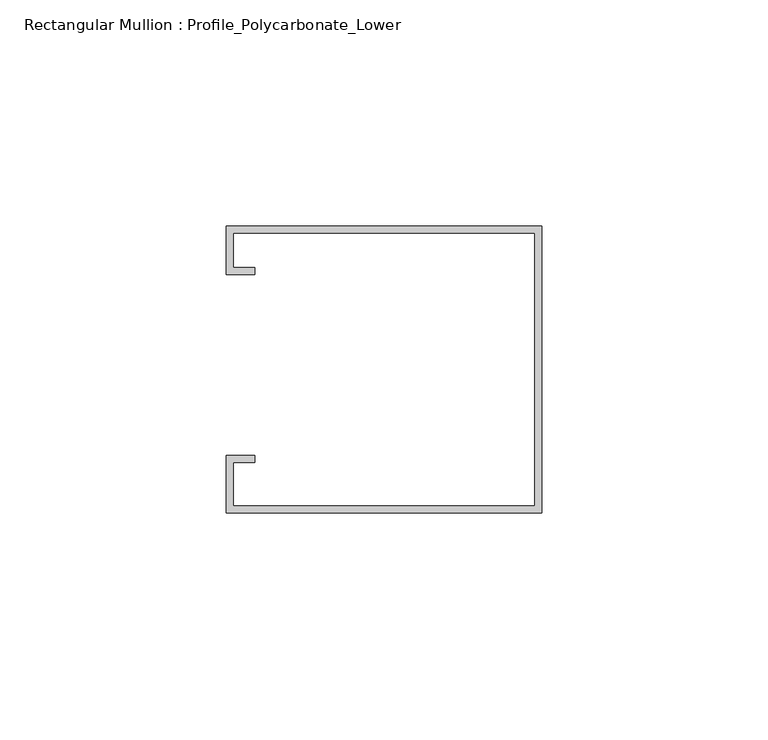
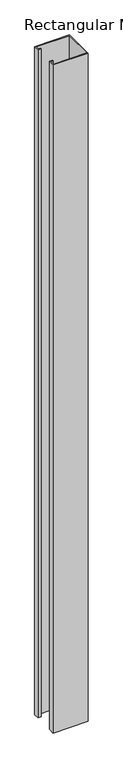
"""IFC4 building model written with IfcOpenShell, lengths in millimetres: member geometry, Rectangular Mullion : Profile_Polycarbonate_Lower."""

from ifc_helpers import new_model, si_unit, frame, origin, place, context, project, spatial, polyline, outline, extrude, source, transform, mapped, element, save


def rectangular_mullion_profile_polycarbonate_lower_301292b8(model_context):
    return source(origin(), model_context, "Body", "SweptSolid", [
        extrude(outline(polyline([(0.0, -32.7), (-69.85, -32.7), (-69.85, -20.0), (-63.5, -20.0), (-63.5, -21.5875), (-68.2625, -21.5875), (-68.2625, -31.1125), (-1.5875, -31.1125), (-1.5875, 29.2125), (-68.2625, 29.2125), (-68.2625, 21.5875), (-63.5, 21.5875), (-63.5, 20.0), (-69.85, 20.0), (-69.85, 30.8), (0.0, 30.8), (0.0, -32.7)])), frame((0.0, 0.0, -1409.7), z_axis=(0.0, 0.0, 1.0), x_axis=(1.0, 0.0, 0.0)), (0.0, 0.0, 1.0), 1409.7),
    ])


if __name__ == "__main__":
    model = new_model("IFC4")
    model_context = context("Model", 3, world=origin())
    ifc_project = project(units=[si_unit("LENGTHUNIT", "METRE", prefix="MILLI")], contexts=[model_context])
    site = spatial("IfcSite", under=ifc_project)
    building = spatial("IfcBuilding", under=site)
    placement = place(None, origin())
    rectangular_mullion_profile_polycarbonate_lower_shape = rectangular_mullion_profile_polycarbonate_lower_301292b8(model_context)
    element("IfcMember", 1, ObjectType="Rectangular Mullion : Profile_Polycarbonate_Lower", at=placement, inside=building, context=model_context, shape_type="MappedRepresentation", body=[
        mapped(rectangular_mullion_profile_polycarbonate_lower_shape, transform((0.0, 0.0, 0.0), x_axis=(1.0, 0.0, 0.0), y_axis=(0.0, 1.0, 0.0), z_axis=(0.0, 0.0, 1.0))),
    ])
    save(model, "model.ifc")

# Revit data of these elements
# Type "Rectangular Mullion : Profile_Polycarbonate_Lower"
#   built-in parameter 1007322 = 0.208333 (stored number, unit not read)
#   built-in parameter 1007321 = 0 (stored number, unit not read)
#   built-in parameter 1007320 = 0.00520833 (stored number, unit not read)
# Element 1 (IfcMember, "Rectangular Mullion : Profile_Polycarbonate_Lower")
#   Materials on its faces: "ALUMINUM PROFILE AT POLYCARBONATE PANEL"
# Materials
#   "ALUMINUM PROFILE AT POLYCARBONATE PANEL": class "Metal", colour RGB 244 244 244, transparency 0, Description = "Aluminum 6061", Cost = 0
